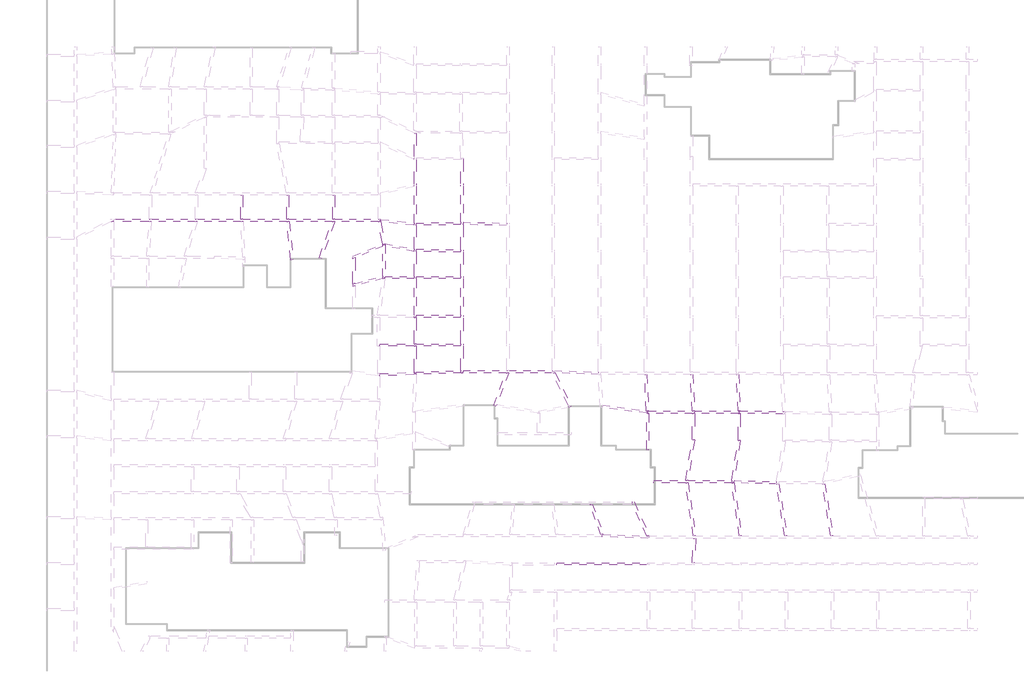
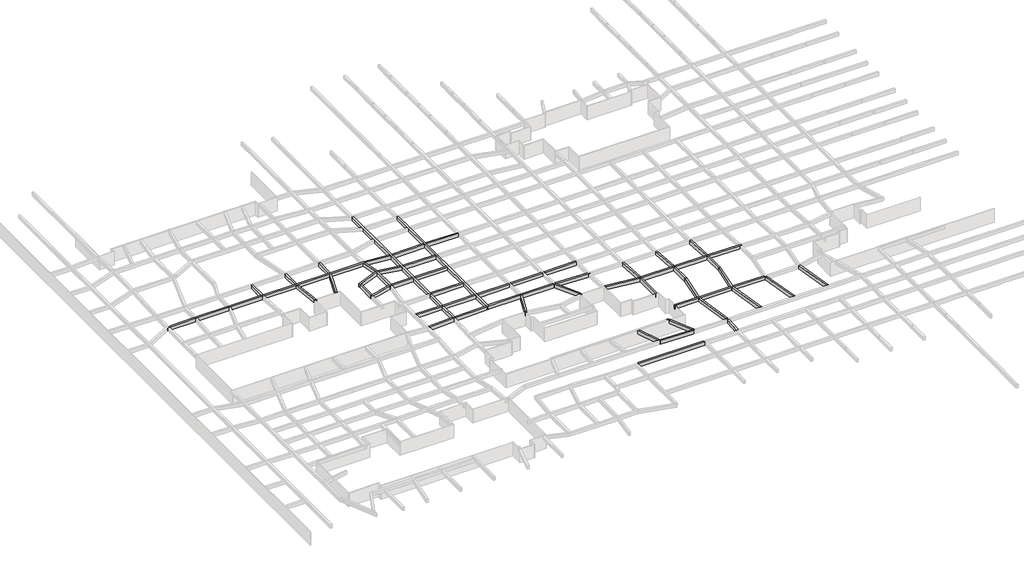
# One storey, part 20 of 45: 53 beams.
"""IFC4 building model written with IfcOpenShell, lengths in millimetres."""

from ifc_helpers import new_model, si_unit, frame, origin, place, context, project, spatial, polyline, outline, extrude, faceted_brep, element, save

model = new_model("IFC4")

# Units and contexts
model_context = context("Model", 3, world=origin())
ifc_project = project(units=[si_unit("LENGTHUNIT", "METRE", prefix="MILLI")], contexts=[model_context])

# Site, building, storey
site = spatial("IfcSite", under=ifc_project)
building = spatial("IfcBuilding", under=site)
storey = spatial("IfcBuildingStorey", under=building, Name="户型图", Elevation=0.0)

# Beams
placement = place(None, origin())
element("IfcBeam", 1, ObjectType="混凝土 - 矩形梁 : KL_beam", at=placement, inside=storey, context=model_context, shape_type="Brep", body=[
    faceted_brep([(-98412.8771817, -3306.533538, 3300.0), (-98412.8771817, -3089.2020745, 3300.0), (-98412.8771817, -2926.5480751, 3300.0), (-98412.8771817, -2906.533538, 3300.0), (-98812.8771817, -2906.533538, 3300.0), (-106143.1610176, -2906.533538, 3300.0), (-106543.1610176, -2906.533538, 3300.0), (-113943.1610176, -2906.533538, 3300.0), (-114343.1610176, -2906.533538, 3300.0), (-121743.1610176, -2906.533538, 3300.0), (-122143.1610176, -2906.533538, 3300.0), (-129467.9283627, -2906.533538, 3300.0), (-129867.9283627, -2906.533538, 3300.0), (-137267.9283627, -2906.533538, 3300.0), (-137667.9283627, -2906.533538, 3300.0), (-143362.5840071, -2906.533538, 3300.0), (-144147.6282093, -3306.533538, 3300.0), (-144104.0852782, -3306.533538, 3300.0), (-143704.0852782, -3306.533538, 3300.0), (-137682.4021047, -3306.533538, 3300.0), (-137281.4253454, -3306.533538, 3300.0), (-129938.2128502, -3306.533538, 3300.0), (-129519.9361477, -3306.533538, 3300.0), (-122132.953931, -3306.533538, 3300.0), (-121732.4049926, -3306.533538, 3300.0), (-114323.2418265, -3306.533538, 3300.0), (-113921.0385147, -3306.533538, 3300.0), (-106625.5164731, -3306.533538, 3300.0), (-106201.4956125, -3306.533538, 3300.0), (-98778.0584965, -3306.533538, 3300.0), (-98412.8771817, -2906.533538, 2500.0), (-98812.8771817, -2906.533538, 2500.0), (-106143.1610176, -2906.533538, 2500.0), (-106543.1610176, -2906.533538, 2500.0), (-113943.1610176, -2906.533538, 2500.0), (-114343.1610176, -2906.533538, 2500.0), (-121743.1610176, -2906.533538, 2500.0), (-122143.1610176, -2906.533538, 2500.0), (-129467.9283627, -2906.533538, 2500.0), (-129867.9283627, -2906.533538, 2500.0), (-137267.9283627, -2906.533538, 2500.0), (-137667.9283627, -2906.533538, 2500.0), (-143362.5840071, -2906.533538, 2500.0), (-98412.8771817, -2926.5480751, 2500.0), (-98412.8771817, -3089.2020745, 2500.0), (-98412.8771817, -3306.533538, 2500.0), (-98778.0584965, -3306.533538, 2500.0), (-106201.4956125, -3306.533538, 2500.0), (-106625.5164731, -3306.533538, 2500.0), (-113921.0385147, -3306.533538, 2500.0), (-114323.2418265, -3306.533538, 2500.0), (-121732.4049926, -3306.533538, 2500.0), (-122132.953931, -3306.533538, 2500.0), (-129519.9361477, -3306.533538, 2500.0), (-129938.2128502, -3306.533538, 2500.0), (-137281.4253454, -3306.533538, 2500.0), (-137682.4021047, -3306.533538, 2500.0), (-143704.0852782, -3306.533538, 2500.0), (-144104.0852782, -3306.533538, 2500.0), (-144147.6282093, -3306.533538, 2500.0)], [[[0, 1, 2, 3, 4, 5, 6, 7, 8, 9, 10, 11, 12, 13, 14, 15, 16, 17, 18, 19, 20, 21, 22, 23, 24, 25, 26, 27, 28, 29]], [[3, 30, 31, 32, 33, 34, 35, 36, 37, 38, 39, 40, 41, 42, 15, 14, 13, 12, 11, 10, 9, 8, 7, 6, 5, 4]], [[30, 43, 44, 45, 46, 47, 48, 49, 50, 51, 52, 53, 54, 55, 56, 57, 58, 59, 42, 41, 40, 39, 38, 37, 36, 35, 34, 33, 32, 31]], [[45, 0, 29, 28, 27, 26, 25, 24, 23, 22, 21, 20, 19, 18, 17, 16, 59, 58, 57, 56, 55, 54, 53, 52, 51, 50, 49, 48, 47, 46]], [[16, 15, 42, 59]], [[3, 2, 1, 0, 45, 44, 43, 30]]]),
])
element("IfcBeam", 2, ObjectType="混凝土 - 矩形梁 : KL_beam", at=placement, inside=storey, context=model_context, shape_type="Brep", body=[
    faceted_brep([(-92291.6701424, 11700.217385, 3300.0), (-92534.6339278, 11700.217385, 3300.0), (-92691.6701424, 11770.1344124, 3300.0), (-92691.6701424, 7708.1903778, 3300.0), (-92691.6701424, 7270.3358664, 3300.0), (-92691.6701424, 3075.9119134, 3300.0), (-92691.6701424, 2663.6664617, 3300.0), (-92691.6701424, -3530.9179057, 3300.0), (-92691.6701424, -3933.1435393, 3300.0), (-92691.6701424, -7966.4140235, 3300.0), (-92691.6701424, -8373.1172498, 3300.0), (-92691.6701424, -12606.533538, 3300.0), (-92691.6701424, -13006.533538, 3300.0), (-92691.6701424, -19206.533538, 3300.0), (-92691.6701424, -19606.533538, 3300.0), (-92291.6701424, -19606.533538, 3300.0), (-92291.6701424, -19566.2432363, 3300.0), (-92291.6701424, -19166.2432363, 3300.0), (-92291.6701424, -13006.533538, 3300.0), (-92291.6701424, -12606.533538, 3300.0), (-92291.6701424, -8372.0681142, 3300.0), (-92291.6701424, -7972.007183, 3300.0), (-92291.6701424, -3949.6812515, 3300.0), (-92291.6701424, -3549.6203203, 3300.0), (-92291.6701424, 2719.5822838, 3300.0), (-92291.6701424, 3119.5822838, 3300.0), (-92291.6701424, 7200.318112, 3300.0), (-92291.6701424, 7600.318112, 3300.0), (-92691.6701424, 11770.1344124, 2500.0), (-92691.6701424, 7708.1903778, 2500.0), (-92691.6701424, 7270.3358664, 2500.0), (-92691.6701424, 3075.9119134, 2500.0), (-92691.6701424, 2663.6664617, 2500.0), (-92691.6701424, -3530.9179057, 2500.0), (-92691.6701424, -3933.1435393, 2500.0), (-92691.6701424, -7966.4140235, 2500.0), (-92691.6701424, -8373.1172498, 2500.0), (-92691.6701424, -12606.533538, 2500.0), (-92691.6701424, -13006.533538, 2500.0), (-92691.6701424, -19206.533538, 2500.0), (-92691.6701424, -19606.533538, 2500.0), (-92534.6339278, 11700.217385, 2500.0), (-92291.6701424, 11700.217385, 2500.0), (-92291.6701424, 7600.318112, 2500.0), (-92291.6701424, 7200.318112, 2500.0), (-92291.6701424, 3119.5822838, 2500.0), (-92291.6701424, 2719.5822838, 2500.0), (-92291.6701424, -3549.6203203, 2500.0), (-92291.6701424, -3949.6812515, 2500.0), (-92291.6701424, -7972.007183, 2500.0), (-92291.6701424, -8372.0681142, 2500.0), (-92291.6701424, -12606.533538, 2500.0), (-92291.6701424, -13006.533538, 2500.0), (-92291.6701424, -19166.2432363, 2500.0), (-92291.6701424, -19566.2432363, 2500.0), (-92291.6701424, -19606.533538, 2500.0)], [[[0, 1, 2, 3, 4, 5, 6, 7, 8, 9, 10, 11, 12, 13, 14, 15, 16, 17, 18, 19, 20, 21, 22, 23, 24, 25, 26, 27]], [[2, 28, 29, 30, 31, 32, 33, 34, 35, 36, 37, 38, 39, 40, 14, 13, 12, 11, 10, 9, 8, 7, 6, 5, 4, 3]], [[41, 42, 43, 44, 45, 46, 47, 48, 49, 50, 51, 52, 53, 54, 55, 40, 39, 38, 37, 36, 35, 34, 33, 32, 31, 30, 29, 28]], [[42, 0, 27, 26, 25, 24, 23, 22, 21, 20, 19, 18, 17, 16, 15, 55, 54, 53, 52, 51, 50, 49, 48, 47, 46, 45, 44, 43]], [[41, 1, 0, 42]], [[1, 41, 28, 2]], [[15, 14, 40, 55]]]),
])
element("IfcBeam", 3, ObjectType="混凝土 - 矩形梁 : KL_beam", at=placement, inside=storey, context=model_context, shape_type="SweptSolid", body=[
    extrude(outline(polyline([(-121743.1610176, -2906.533538), (-122143.1610176, -2906.533538), (-122143.1610176, 1193.466462), (-121743.1610176, 1193.466462), (-121743.1610176, -2906.533538)])), frame((0.0, 0.0, 2500.0), z_axis=(0.0, 0.0, 1.0), x_axis=(1.0, 0.0, 0.0)), (0.0, 0.0, 1.0), 800.0),
])
element("IfcBeam", 4, ObjectType="混凝土 - 矩形梁 : KL_beam", at=placement, inside=storey, context=model_context, shape_type="SweptSolid", body=[
    extrude(outline(polyline([(-113943.1610176, -2906.533538), (-114343.1610176, -2906.533538), (-114343.1610176, 1193.466462), (-113943.1610176, 1193.466462), (-113943.1610176, -2906.533538)])), frame((0.0, 0.0, 2500.0), z_axis=(0.0, 0.0, 1.0), x_axis=(1.0, 0.0, 0.0)), (0.0, 0.0, 1.0), 800.0),
])
element("IfcBeam", 5, ObjectType="混凝土 - 矩形梁 : KL_beam", at=placement, inside=storey, context=model_context, shape_type="SweptSolid", body=[
    extrude(outline(polyline([(-106143.1610176, -2906.533538), (-106543.1610176, -2906.533538), (-106543.1610176, 1193.466462), (-106143.1610176, 1193.466462), (-106143.1610176, -2906.533538)])), frame((0.0, 0.0, 2500.0), z_axis=(0.0, 0.0, 1.0), x_axis=(1.0, 0.0, 0.0)), (0.0, 0.0, 1.0), 800.0),
])
element("IfcBeam", 6, ObjectType="混凝土 - 矩形梁 : KL_beam", at=placement, inside=storey, context=model_context, shape_type="SweptSolid", body=[
    extrude(outline(polyline([(-113240.416887, -9782.2157591), (-113638.2256451, -9824.0271444), (-114323.2418265, -3306.533538), (-113921.0385147, -3306.533538), (-113240.416887, -9782.2157591)])), frame((0.0, 0.0, 2500.0), z_axis=(0.0, 0.0, 1.0), x_axis=(1.0, 0.0, 0.0)), (0.0, 0.0, 1.0), 800.0),
])
element("IfcBeam", 7, ObjectType="混凝土 - 矩形梁 : KL_beam", at=placement, inside=storey, context=model_context, shape_type="SweptSolid", body=[
    extrude(outline(polyline([(-108410.7299112, -9587.6722396), (-108788.0698368, -9454.9523069), (-106625.5164731, -3306.533538), (-106201.4956125, -3306.533538), (-108410.7299112, -9587.6722396)])), frame((0.0, 0.0, 2500.0), z_axis=(0.0, 0.0, 1.0), x_axis=(1.0, 0.0, 0.0)), (0.0, 0.0, 1.0), 800.0),
])
element("IfcBeam", 8, ObjectType="混凝土 - 矩形梁 : KL_beam", at=placement, inside=storey, context=model_context, shape_type="Brep", body=[
    faceted_brep([(-97610.1601463, -7209.73689, 3300.0), (-97639.9689694, -7056.7212093, 3300.0), (-98365.2258689, -3333.8074395, 3300.0), (-98412.8771817, -3089.2020745, 3300.0), (-98412.8771817, -3306.533538, 3300.0), (-98778.0584965, -3306.533538, 3300.0), (-98038.0080665, -7105.3859697, 3300.0), (-98010.1601463, -7248.3358759, 3300.0), (-98778.0584965, -3306.533538, 2500.0), (-98038.0080665, -7105.3859697, 2500.0), (-98010.1601463, -7248.3358759, 2500.0), (-98412.8771817, -3306.533538, 2500.0), (-98412.8771817, -3089.2020745, 2500.0), (-98365.2258689, -3333.8074395, 2500.0), (-97639.9689694, -7056.7212093, 2500.0), (-97610.1601463, -7209.73689, 2500.0)], [[[0, 1, 2, 3, 4, 5, 6, 7]], [[7, 6, 5, 8, 9, 10]], [[10, 9, 8, 11, 12, 13, 14, 15]], [[3, 2, 1, 0, 15, 14, 13, 12]], [[4, 11, 8, 5]], [[11, 4, 3, 12]], [[0, 7, 10, 15]]]),
])
element("IfcBeam", 9, ObjectType="混凝土 - 矩形梁 : KL_beam", at=placement, inside=storey, context=model_context, shape_type="Brep", body=[
    faceted_brep([(-97610.1601463, -7209.73689, 3300.0), (-98010.1601463, -7248.3358759, 3300.0), (-98010.1601463, -7525.5485767, 3300.0), (-98010.1601463, -12553.0681404, 3300.0), (-98010.1601463, -12967.1786125, 3300.0), (-97610.1601463, -12859.9989355, 3300.0), (-97610.1601463, -12606.533538, 3300.0), (-97610.1601463, -7468.9044749, 3300.0), (-97610.1601463, -7363.9380863, 3300.0), (-98010.1601463, -7248.3358759, 2500.0), (-98010.1601463, -7525.5485767, 2500.0), (-98010.1601463, -12553.0681404, 2500.0), (-98010.1601463, -12967.1786125, 2500.0), (-97610.1601463, -7209.73689, 2500.0), (-97610.1601463, -7363.9380863, 2500.0), (-97610.1601463, -7468.9044749, 2500.0), (-97610.1601463, -12606.533538, 2500.0), (-97610.1601463, -12859.9989355, 2500.0)], [[[0, 1, 2, 3, 4, 5, 6, 7, 8]], [[1, 9, 10, 11, 12, 4, 3, 2]], [[9, 13, 14, 15, 16, 17, 12, 11, 10]], [[13, 0, 8, 7, 6, 5, 17, 16, 15, 14]], [[0, 13, 9, 1]], [[5, 4, 12, 17]]]),
])
element("IfcBeam", 10, ObjectType="混凝土 - 矩形梁 : KL_beam", at=placement, inside=storey, context=model_context, shape_type="Brep", body=[
    faceted_brep([(-98010.1601463, -7248.3358759, 3300.0), (-98038.0080665, -7105.3859697, 3300.0), (-103109.6713464, -9154.4709434, 3300.0), (-103109.6713464, -9585.8848405, 3300.0), (-102709.6713464, -9424.2743501, 3300.0), (-98010.1601463, -7525.5485767, 3300.0), (-98038.0080665, -7105.3859697, 2500.0), (-103109.6713464, -9154.4709434, 2500.0), (-98010.1601463, -7248.3358759, 2500.0), (-98010.1601463, -7525.5485767, 2500.0), (-102709.6713464, -9424.2743501, 2500.0), (-103109.6713464, -9585.8848405, 2500.0)], [[[0, 1, 2, 3, 4, 5]], [[1, 6, 7, 2]], [[6, 8, 9, 10, 11, 7]], [[3, 11, 10, 9, 5, 4]], [[1, 0, 8, 6]], [[0, 5, 9, 8]], [[3, 2, 7, 11]]]),
    faceted_brep([(-97582.312226, -7352.6867962, 3300.0), (-97582.312226, -7352.6867962, 2500.0), (-97610.1601463, -7209.73689, 2500.0), (-97610.1601463, -7209.73689, 3300.0), (-97610.1601463, -7363.9380863, 3300.0), (-97610.1601463, -7363.9380863, 2500.0)], [[[0, 1, 2, 3]], [[4, 3, 2, 5]], [[0, 3, 4]], [[2, 1, 5]], [[1, 0, 4, 5]]]),
])
element("IfcBeam", 11, ObjectType="混凝土 - 矩形梁 : KL_beam", at=placement, inside=storey, context=model_context, shape_type="Brep", body=[
    faceted_brep([(-103109.6713464, -13919.4780482, 3300.0), (-103006.1437284, -14305.8483787, 3300.0), (-102709.6713464, -14226.4088434, 3300.0), (-98050.230566, -12977.9154491, 3300.0), (-98010.1601463, -12967.1786125, 3300.0), (-98010.1601463, -12553.0681404, 3300.0), (-102709.6713464, -13812.2983712, 3300.0), (-103109.6713464, -13919.4780482, 2500.0), (-98010.1601463, -12553.0681404, 2500.0), (-102709.6713464, -13812.2983712, 2500.0), (-103006.1437284, -14305.8483787, 2500.0), (-98010.1601463, -12967.1786125, 2500.0), (-98050.230566, -12977.9154491, 2500.0), (-102709.6713464, -14226.4088434, 2500.0)], [[[0, 1, 2, 3, 4, 5, 6]], [[7, 0, 6, 5, 8, 9]], [[10, 7, 9, 8, 11, 12, 13]], [[1, 10, 13, 12, 11, 4, 3, 2]], [[5, 4, 11, 8]], [[1, 0, 7, 10]]]),
])
element("IfcBeam", 12, ObjectType="混凝土 - 矩形梁 : KL_beam", at=placement, inside=storey, context=model_context, shape_type="SweptSolid", body=[
    extrude(outline(polyline([(-103109.6713464, -13919.4780482), (-103109.6713464, -9585.8848405), (-102709.6713464, -9424.2743501), (-102709.6713464, -13812.2983712), (-103109.6713464, -13919.4780482)])), frame((0.0, 0.0, 2500.0), z_axis=(0.0, 0.0, 1.0), x_axis=(1.0, 0.0, 0.0)), (0.0, 0.0, 1.0), 800.0),
])
element("IfcBeam", 13, ObjectType="混凝土 - 矩形梁 : KL_beam", at=placement, inside=storey, context=model_context, shape_type="Brep", body=[
    faceted_brep([(-98010.1601463, -13006.533538, 3300.0), (-97650.3215471, -13006.533538, 3300.0), (-92691.6701424, -13006.533538, 3300.0), (-92691.6701424, -12606.533538, 3300.0), (-97610.1601463, -12606.533538, 3300.0), (-97610.1601463, -12859.9989355, 3300.0), (-98010.1601463, -12967.1786125, 3300.0), (-92691.6701424, -12606.533538, 2500.0), (-97610.1601463, -12606.533538, 2500.0), (-92691.6701424, -13006.533538, 2500.0), (-97650.3215471, -13006.533538, 2500.0), (-98010.1601463, -13006.533538, 2500.0), (-98010.1601463, -12967.1786125, 2500.0), (-97610.1601463, -12859.9989355, 2500.0)], [[[0, 1, 2, 3, 4, 5, 6]], [[3, 7, 8, 4]], [[9, 10, 11, 12, 13, 8, 7]], [[0, 11, 10, 9, 2, 1]], [[11, 0, 6, 12]], [[3, 2, 9, 7]], [[5, 13, 12, 6]], [[13, 5, 4, 8]]]),
])
element("IfcBeam", 14, ObjectType="混凝土 - 矩形梁 : KL_beam", at=placement, inside=storey, context=model_context, shape_type="Brep", body=[
    faceted_brep([(-92691.6701424, -8373.1172498, 3300.0), (-92691.6701424, -7966.4140235, 3300.0), (-97639.9689694, -7056.7212093, 3300.0), (-97610.1601463, -7209.73689, 3300.0), (-97582.312226, -7352.6867962, 3300.0), (-97610.1601463, -7363.9380863, 3300.0), (-97610.1601463, -7468.9044749, 3300.0), (-92691.6701424, -7966.4140235, 2500.0), (-97639.9689694, -7056.7212093, 2500.0), (-92691.6701424, -8373.1172498, 2500.0), (-97610.1601463, -7468.9044749, 2500.0), (-97610.1601463, -7363.9380863, 2500.0), (-97582.312226, -7352.6867962, 2500.0), (-97610.1601463, -7209.73689, 2500.0)], [[[0, 1, 2, 3, 4, 5, 6]], [[1, 7, 8, 2]], [[7, 9, 10, 11, 12, 13, 8]], [[9, 0, 6, 10]], [[1, 0, 9, 7]], [[2, 8, 13, 12, 4, 3]], [[10, 6, 5, 11]], [[4, 12, 11, 5]]]),
])
element("IfcBeam", 15, ObjectType="混凝土 - 矩形梁 : KL_beam", at=placement, inside=storey, context=model_context, shape_type="SweptSolid", body=[
    extrude(outline(polyline([(-98412.8771817, -2926.5480751), (-92691.6701424, -3530.9179057), (-92691.6701424, -3933.1435393), (-98365.2258689, -3333.8074395), (-98412.8771817, -3089.2020745), (-98412.8771817, -2926.5480751)])), frame((0.0, 0.0, 2500.0), z_axis=(0.0, 0.0, 1.0), x_axis=(1.0, 0.0, 0.0)), (0.0, 0.0, 1.0), 800.0),
])
element("IfcBeam", 16, ObjectType="混凝土 - 矩形梁 : KL_beam", at=placement, inside=storey, context=model_context, shape_type="Brep", body=[
    faceted_brep([(-84386.4058027, 7406.4496764, 3300.0), (-84786.4058027, 7399.4676504, 3300.0), (-84786.4058027, 7200.318112, 3300.0), (-84786.4058027, 3119.5822838, 3300.0), (-84786.4058027, 2719.5822838, 3300.0), (-84786.4058027, -3418.615444, 3300.0), (-84786.4058027, -3818.6763752, 3300.0), (-84786.4058027, -8103.0120594, 3300.0), (-84786.4058027, -8503.0729906, 3300.0), (-84786.4058027, -12606.533538, 3300.0), (-84786.4058027, -13006.533538, 3300.0), (-84786.4058027, -19166.2432363, 3300.0), (-84786.4058027, -19566.2432363, 3300.0), (-84786.4058027, -24066.2432363, 3300.0), (-84786.4058027, -24466.2432363, 3300.0), (-84786.4058027, -28603.7362156, 3300.0), (-84786.4058027, -29003.9680843, 3300.0), (-84583.0013827, -28997.0413366, 3300.0), (-84386.4058027, -28990.3464576, 3300.0), (-84386.4058027, -28597.0413366, 3300.0), (-84386.4058027, -24466.2432363, 3300.0), (-84386.4058027, -24066.2432363, 3300.0), (-84386.4058027, -19666.2432363, 3300.0), (-84386.4058027, -19266.2432363, 3300.0), (-84386.4058027, -13006.533538, 3300.0), (-84386.4058027, -12606.533538, 3300.0), (-84386.4058027, -8506.533538, 3300.0), (-84386.4058027, -8106.533538, 3300.0), (-84386.4058027, -3818.6763752, 3300.0), (-84386.4058027, -3418.615444, 3300.0), (-84386.4058027, 2719.5822838, 3300.0), (-84386.4058027, 3119.5822838, 3300.0), (-84386.4058027, 7200.318112, 3300.0), (-84786.4058027, 7399.4676504, 2500.0), (-84786.4058027, 7200.318112, 2500.0), (-84786.4058027, 3119.5822838, 2500.0), (-84786.4058027, 2719.5822838, 2500.0), (-84786.4058027, -3418.615444, 2500.0), (-84786.4058027, -3818.6763752, 2500.0), (-84786.4058027, -8103.0120594, 2500.0), (-84786.4058027, -8503.0729906, 2500.0), (-84786.4058027, -12606.533538, 2500.0), (-84786.4058027, -13006.533538, 2500.0), (-84786.4058027, -19166.2432363, 2500.0), (-84786.4058027, -19566.2432363, 2500.0), (-84786.4058027, -24066.2432363, 2500.0), (-84786.4058027, -24466.2432363, 2500.0), (-84786.4058027, -28603.7362156, 2500.0), (-84786.4058027, -29003.9680843, 2500.0), (-84386.4058027, 7406.4496764, 2500.0), (-84386.4058027, 7200.318112, 2500.0), (-84386.4058027, 3119.5822838, 2500.0), (-84386.4058027, 2719.5822838, 2500.0), (-84386.4058027, -3418.615444, 2500.0), (-84386.4058027, -3818.6763752, 2500.0), (-84386.4058027, -8106.533538, 2500.0), (-84386.4058027, -8506.533538, 2500.0), (-84386.4058027, -12606.533538, 2500.0), (-84386.4058027, -13006.533538, 2500.0), (-84386.4058027, -19266.2432363, 2500.0), (-84386.4058027, -19666.2432363, 2500.0), (-84386.4058027, -24066.2432363, 2500.0), (-84386.4058027, -24466.2432363, 2500.0), (-84386.4058027, -28597.0413366, 2500.0), (-84386.4058027, -28990.3464576, 2500.0), (-84583.0013827, -28997.0413366, 2500.0)], [[[0, 1, 2, 3, 4, 5, 6, 7, 8, 9, 10, 11, 12, 13, 14, 15, 16, 17, 18, 19, 20, 21, 22, 23, 24, 25, 26, 27, 28, 29, 30, 31, 32]], [[1, 33, 34, 35, 36, 37, 38, 39, 40, 41, 42, 43, 44, 45, 46, 47, 48, 16, 15, 14, 13, 12, 11, 10, 9, 8, 7, 6, 5, 4, 3, 2]], [[33, 49, 50, 51, 52, 53, 54, 55, 56, 57, 58, 59, 60, 61, 62, 63, 64, 65, 48, 47, 46, 45, 44, 43, 42, 41, 40, 39, 38, 37, 36, 35, 34]], [[49, 0, 32, 31, 30, 29, 28, 27, 26, 25, 24, 23, 22, 21, 20, 19, 18, 64, 63, 62, 61, 60, 59, 58, 57, 56, 55, 54, 53, 52, 51, 50]], [[0, 49, 33, 1]], [[18, 17, 16, 48, 65, 64]]]),
])
element("IfcBeam", 17, ObjectType="混凝土 - 矩形梁 : KL_beam", at=placement, inside=storey, context=model_context, shape_type="SweptSolid", body=[
    extrude(outline(polyline([(-92291.6701424, -3949.6812515), (-92291.6701424, -3549.6203203), (-84786.4058027, -3418.615444), (-84786.4058027, -3818.6763752), (-92291.6701424, -3949.6812515)])), frame((0.0, 0.0, 2500.0), z_axis=(0.0, 0.0, 1.0), x_axis=(1.0, 0.0, 0.0)), (0.0, 0.0, 1.0), 800.0),
])
element("IfcBeam", 18, ObjectType="混凝土 - 矩形梁 : KL_beam", at=placement, inside=storey, context=model_context, shape_type="SweptSolid", body=[
    extrude(outline(polyline([(-76974.0592951, -3547.9984335), (-76974.0592951, -3948.0593648), (-84386.4058027, -3818.6763752), (-84386.4058027, -3418.615444), (-76974.0592951, -3547.9984335)])), frame((0.0, 0.0, 2500.0), z_axis=(0.0, 0.0, 1.0), x_axis=(1.0, 0.0, 0.0)), (0.0, 0.0, 1.0), 800.0),
])
element("IfcBeam", 19, ObjectType="混凝土 - 矩形梁 : KL_beam", at=placement, inside=storey, context=model_context, shape_type="SweptSolid", body=[
    extrude(outline(polyline([(-92291.6701424, -8372.0681142), (-92291.6701424, -7972.007183), (-84786.4058027, -8103.0120594), (-84786.4058027, -8503.0729906), (-92291.6701424, -8372.0681142)])), frame((0.0, 0.0, 2500.0), z_axis=(0.0, 0.0, 1.0), x_axis=(1.0, 0.0, 0.0)), (0.0, 0.0, 1.0), 800.0),
])
element("IfcBeam", 20, ObjectType="混凝土 - 矩形梁 : KL_beam", at=placement, inside=storey, context=model_context, shape_type="SweptSolid", body=[
    extrude(outline(polyline([(-92291.6701424, -13006.533538), (-92291.6701424, -12606.533538), (-84786.4058027, -12606.533538), (-84786.4058027, -13006.533538), (-92291.6701424, -13006.533538)])), frame((0.0, 0.0, 2500.0), z_axis=(0.0, 0.0, 1.0), x_axis=(1.0, 0.0, 0.0)), (0.0, 0.0, 1.0), 800.0),
])
element("IfcBeam", 21, ObjectType="混凝土 - 矩形梁 : KL_beam", at=placement, inside=storey, context=model_context, shape_type="SweptSolid", body=[
    extrude(outline(polyline([(-92291.6701424, -19566.2432363), (-92291.6701424, -19166.2432363), (-84786.4058027, -19166.2432363), (-84786.4058027, -19566.2432363), (-92291.6701424, -19566.2432363)])), frame((0.0, 0.0, 2500.0), z_axis=(0.0, 0.0, 1.0), x_axis=(1.0, 0.0, 0.0)), (0.0, 0.0, 1.0), 800.0),
])
element("IfcBeam", 22, ObjectType="混凝土 - 矩形梁 : KL_beam", at=placement, inside=storey, context=model_context, shape_type="SweptSolid", body=[
    extrude(outline(polyline([(-92691.5379725, -19606.533538), (-92291.5379725, -19606.533538), (-92291.5379725, -24066.2432363), (-92691.5379725, -24066.2432363), (-92691.5379725, -19606.533538)])), frame((0.0, 0.0, 2500.0), z_axis=(0.0, 0.0, 1.0), x_axis=(1.0, 0.0, 0.0)), (0.0, 0.0, 1.0), 800.0),
])
element("IfcBeam", 23, ObjectType="混凝土 - 矩形梁 : KL_beam", at=placement, inside=storey, context=model_context, shape_type="Brep", body=[
    faceted_brep([(-98551.6884215, -24066.2432363, 3300.0), (-98551.6884215, -24466.2432363, 3300.0), (-98489.6882512, -24466.2432363, 3300.0), (-92691.5379725, -24466.2432363, 3300.0), (-92291.5379725, -24466.2432363, 3300.0), (-84786.4058027, -24466.2432363, 3300.0), (-84786.4058027, -24066.2432363, 3300.0), (-92291.5379725, -24066.2432363, 3300.0), (-92691.5379725, -24066.2432363, 3300.0), (-98551.6884215, -24066.2432363, 2500.0), (-84786.4058027, -24066.2432363, 2500.0), (-92291.5379725, -24066.2432363, 2500.0), (-92691.5379725, -24066.2432363, 2500.0), (-98551.6884215, -24466.2432363, 2500.0), (-84786.4058027, -24466.2432363, 2500.0), (-92291.5379725, -24466.2432363, 2500.0), (-92691.5379725, -24466.2432363, 2500.0), (-98489.6882512, -24466.2432363, 2500.0)], [[[0, 1, 2, 3, 4, 5, 6, 7, 8]], [[9, 0, 8, 7, 6, 10, 11, 12]], [[13, 9, 12, 11, 10, 14, 15, 16, 17]], [[1, 13, 17, 16, 15, 14, 5, 4, 3, 2]], [[1, 0, 9, 13]], [[6, 5, 14, 10]]]),
    faceted_brep([(-61385.2176693, -24066.2432363, 3300.0), (-61385.2176693, -24466.2432363, 3300.0), (-61385.2176693, -24466.2432363, 2500.0), (-61385.2176693, -24066.2432363, 2500.0), (-68859.410716, -24466.2432363, 3300.0), (-68859.410716, -24066.2432363, 3300.0), (-68859.410716, -24066.2432363, 2500.0), (-68859.410716, -24466.2432363, 2500.0)], [[[0, 1, 2, 3]], [[4, 5, 6, 7]], [[1, 0, 5, 4]], [[0, 3, 6, 5]], [[3, 2, 7, 6]], [[2, 1, 4, 7]]]),
    faceted_brep([(-76974.0592951, -24066.2432363, 3300.0), (-76974.0592951, -24466.2432363, 3300.0), (-76974.0592951, -24466.2432363, 2500.0), (-76974.0592951, -24066.2432363, 2500.0), (-84386.4058027, -24466.2432363, 3300.0), (-84386.4058027, -24066.2432363, 3300.0), (-84386.4058027, -24066.2432363, 2500.0), (-84386.4058027, -24466.2432363, 2500.0)], [[[0, 1, 2, 3]], [[4, 5, 6, 7]], [[1, 0, 5, 4]], [[0, 3, 6, 5]], [[3, 2, 7, 6]], [[2, 1, 4, 7]]]),
    faceted_brep([(-76574.0592951, -24466.2432363, 3300.0), (-76574.0592951, -24066.2432363, 3300.0), (-76574.0592951, -24066.2432363, 2500.0), (-76574.0592951, -24466.2432363, 2500.0), (-69259.410716, -24466.2432363, 3300.0), (-69259.410716, -24066.2432363, 3300.0), (-69259.410716, -24066.2432363, 2500.0), (-69259.410716, -24466.2432363, 2500.0)], [[[0, 1, 2, 3]], [[1, 0, 4, 5]], [[2, 1, 5, 6]], [[3, 2, 6, 7]], [[0, 3, 7, 4]], [[5, 4, 7, 6]]]),
])
element("IfcBeam", 24, ObjectType="混凝土 - 矩形梁 : KL_beam", at=placement, inside=storey, context=model_context, shape_type="Brep", body=[
    faceted_brep([(-92691.5379725, -29062.7522233, 3300.0), (-92291.5379725, -29069.7342493, 3300.0), (-92291.5379725, -28859.3164886, 3300.0), (-92291.5379725, -24466.2432363, 3300.0), (-92691.5379725, -24466.2432363, 3300.0), (-92691.5379725, -28874.9728967, 3300.0), (-92691.5379725, -29062.7522233, 2500.0), (-92691.5379725, -24466.2432363, 2500.0), (-92691.5379725, -28874.9728967, 2500.0), (-92291.5379725, -29069.7342493, 2500.0), (-92291.5379725, -24466.2432363, 2500.0), (-92291.5379725, -28859.3164886, 2500.0)], [[[0, 1, 2, 3, 4, 5]], [[6, 0, 5, 4, 7, 8]], [[9, 6, 8, 7, 10, 11]], [[1, 9, 11, 10, 3, 2]], [[4, 3, 10, 7]], [[1, 0, 6, 9]]]),
])
element("IfcBeam", 25, ObjectType="混凝土 - 矩形梁 : KL_beam", at=placement, inside=storey, context=model_context, shape_type="SweptSolid", body=[
    extrude(outline(polyline([(-92691.5379725, -28874.9728967), (-92691.5379725, -29062.7522233), (-92698.9743886, -29275.7033162), (-98489.6882512, -29534.2260627), (-98489.6882512, -29133.8276372), (-92691.5379725, -28874.9728967)])), frame((0.0, 0.0, 2500.0), z_axis=(0.0, 0.0, 1.0), x_axis=(1.0, 0.0, 0.0)), (0.0, 0.0, 1.0), 800.0),
])
element("IfcBeam", 26, ObjectType="混凝土 - 矩形梁 : KL_beam", at=placement, inside=storey, context=model_context, shape_type="Brep", body=[
    faceted_brep([(-84786.4058027, -29003.9680843, 3300.0), (-84786.4058027, -28603.7362156, 3300.0), (-92291.5379725, -28859.3164886, 3300.0), (-92291.5379725, -29069.7342493, 3300.0), (-92298.1056102, -29257.806784, 3300.0), (-92298.1743191, -29259.7743519, 3300.0), (-84786.4058027, -29003.9680843, 2500.0), (-92298.1743191, -29259.7743519, 2500.0), (-84786.4058027, -28603.7362156, 2500.0), (-92298.1056102, -29257.806784, 2500.0), (-92291.5379725, -29069.7342493, 2500.0), (-92291.5379725, -28859.3164886, 2500.0)], [[[0, 1, 2, 3, 4, 5]], [[6, 0, 5, 7]], [[8, 6, 7, 9, 10, 11]], [[1, 8, 11, 2]], [[1, 0, 6, 8]], [[3, 2, 11, 10]], [[7, 5, 4, 3, 10, 9]]]),
])
element("IfcBeam", 27, ObjectType="混凝土 - 矩形梁 : KL_beam", at=placement, inside=storey, context=model_context, shape_type="Brep", body=[
    faceted_brep([(-69259.410716, -28997.0413366, 3300.0), (-69259.410716, -28597.0413366, 3300.0), (-76574.0592951, -28597.0413366, 3300.0), (-76974.0592951, -28597.0413366, 3300.0), (-84386.4058027, -28597.0413366, 3300.0), (-84386.4058027, -28990.3464576, 3300.0), (-84583.0013827, -28997.0413366, 3300.0), (-77065.0611009, -28997.0413366, 3300.0), (-76636.6031034, -28997.0413366, 3300.0), (-69259.410716, -28997.0413366, 2500.0), (-84583.0013827, -28997.0413366, 2500.0), (-77065.0611009, -28997.0413366, 2500.0), (-76636.6031034, -28997.0413366, 2500.0), (-69259.410716, -28597.0413366, 2500.0), (-84386.4058027, -28990.3464576, 2500.0), (-84386.4058027, -28597.0413366, 2500.0), (-76974.0592951, -28597.0413366, 2500.0), (-76574.0592951, -28597.0413366, 2500.0)], [[[0, 1, 2, 3, 4, 5, 6, 7, 8]], [[9, 0, 8, 7, 6, 10, 11, 12]], [[13, 9, 12, 11, 10, 14, 15, 16, 17]], [[1, 13, 17, 16, 15, 4, 3, 2]], [[1, 0, 9, 13]], [[14, 5, 4, 15]], [[5, 14, 10, 6]]]),
])
element("IfcBeam", 28, ObjectType="混凝土 - 矩形梁 : KL_beam", at=placement, inside=storey, context=model_context, shape_type="Brep", body=[
    faceted_brep([(-60985.2176693, -29273.1976575, 3300.0), (-60985.2176693, -29266.2296815, 3300.0), (-60985.2176693, -29259.522509, 3300.0), (-61385.2176693, -29259.522509, 3300.0), (-61375.3451123, -29259.8600307, 3300.0), (-61189.0319378, -29266.2296815, 3300.0), (-60985.2176693, -29273.1976575, 2500.0), (-68733.4619053, -29008.3016795, 3300.0), (-69062.8285047, -28997.0413366, 3300.0), (-69062.8285047, -28997.0413366, 2500.0), (-68733.4619053, -29008.3016795, 2500.0), (-61385.2176693, -29259.522509, 2500.0), (-61375.3451123, -29259.8600307, 2500.0), (-61189.0319378, -29266.2296815, 2500.0), (-60985.2176693, -29259.522509, 2500.0), (-60985.2176693, -29266.2296815, 2500.0), (-68859.410716, -28603.762064, 2500.0), (-68859.410716, -28603.762064, 3300.0), (-61385.2176693, -28859.2888151, 3300.0), (-61385.2176693, -28859.2888151, 2500.0), (-68859.410716, -28997.0413366, 2500.0), (-68859.410716, -28997.0413366, 3300.0)], [[[0, 1, 2, 3, 4, 5]], [[6, 0, 5, 4, 3, 7, 8, 9, 10, 11, 12, 13]], [[14, 15, 6, 13, 12, 11]], [[16, 17, 18, 19]], [[0, 6, 15, 14, 2, 1]], [[20, 21, 17, 16]], [[21, 20, 9, 8]], [[3, 11, 19, 18]], [[11, 3, 2, 14]], [[17, 21, 8, 7, 3, 18]], [[20, 16, 19, 11, 10, 9]]]),
])
element("IfcBeam", 29, ObjectType="混凝土 - 矩形梁 : KL_beam", at=placement, inside=storey, context=model_context, shape_type="Brep", body=[
    faceted_brep([(-45074.9115482, -35866.2296815, 3300.0), (-45074.9115482, -35466.2296815, 3300.0), (-45475.4604866, -35466.2296815, 3300.0), (-52835.3253588, -35466.2296815, 3300.0), (-53012.1394728, -35466.2296815, 3300.0), (-53037.651896, -35866.2296815, 3300.0), (-52825.1182721, -35866.2296815, 3300.0), (-45464.7044616, -35866.2296815, 3300.0), (-45074.9115482, -35866.2296815, 2500.0), (-53037.651896, -35866.2296815, 2500.0), (-52825.1182721, -35866.2296815, 2500.0), (-45464.7044616, -35866.2296815, 2500.0), (-45074.9115482, -35466.2296815, 2500.0), (-53012.1394728, -35466.2296815, 2500.0), (-52835.3253588, -35466.2296815, 2500.0), (-45475.4604866, -35466.2296815, 2500.0)], [[[0, 1, 2, 3, 4, 5, 6, 7]], [[8, 0, 7, 6, 5, 9, 10, 11]], [[12, 8, 11, 10, 9, 13, 14, 15]], [[1, 12, 15, 14, 13, 4, 3, 2]], [[1, 0, 8, 12]], [[4, 13, 9, 5]]]),
])
element("IfcBeam", 30, ObjectType="混凝土 - 矩形梁 : KL_beam", at=placement, inside=storey, context=model_context, shape_type="Brep", body=[
    faceted_brep([(-37472.2975115, -35866.2296815, 3300.0), (-37469.7442944, -35466.2296815, 3300.0), (-37678.745911, -35466.2296815, 3300.0), (-45074.9115482, -35466.2296815, 3300.0), (-45053.9484365, -35866.2296815, 3300.0), (-37667.9878566, -35866.2296815, 3300.0), (-37472.2975115, -35866.2296815, 2500.0), (-45053.9484365, -35866.2296815, 2500.0), (-37667.9878566, -35866.2296815, 2500.0), (-37469.7442944, -35466.2296815, 2500.0), (-45074.9115482, -35466.2296815, 2500.0), (-37678.745911, -35466.2296815, 2500.0)], [[[0, 1, 2, 3, 4, 5]], [[6, 0, 5, 4, 7, 8]], [[9, 6, 8, 7, 10, 11]], [[1, 9, 11, 10, 3, 2]], [[1, 0, 6, 9]], [[4, 3, 10, 7]]]),
])
element("IfcBeam", 31, ObjectType="混凝土 - 矩形梁 : KL_beam", at=placement, inside=storey, context=model_context, shape_type="Brep", body=[
    faceted_brep([(-29669.6887336, -35565.8099149, 3300.0), (-30070.5058465, -35560.6928409, 3300.0), (-37278.0687283, -35468.6767279, 3300.0), (-37469.7442944, -35466.2296815, 3300.0), (-37472.2975115, -35866.2296815, 3300.0), (-37267.9878566, -35868.8380223, 3300.0), (-30059.6078619, -35960.8645671, 3300.0), (-29674.7949597, -35965.7773217, 3300.0), (-37472.2975115, -35866.2296815, 2500.0), (-37267.9878566, -35868.8380223, 2500.0), (-30059.6078619, -35960.8645671, 2500.0), (-29674.7949597, -35965.7773217, 2500.0), (-37469.7442944, -35466.2296815, 2500.0), (-37278.0687283, -35468.6767279, 2500.0), (-30070.5058465, -35560.6928409, 2500.0), (-29669.6887336, -35565.8099149, 2500.0)], [[[0, 1, 2, 3, 4, 5, 6, 7]], [[7, 6, 5, 4, 8, 9, 10, 11]], [[11, 10, 9, 8, 12, 13, 14, 15]], [[3, 2, 1, 0, 15, 14, 13, 12]], [[3, 12, 8, 4]], [[0, 7, 11, 15]]]),
])
element("IfcBeam", 32, ObjectType="混凝土 - 矩形梁 : KL_beam", at=placement, inside=storey, context=model_context, shape_type="SweptSolid", body=[
    extrude(outline(polyline([(-37278.0687283, -35468.6767279), (-37469.7442944, -35466.2296815), (-37678.745911, -35466.2296815), (-38003.6741425, -29266.2296815), (-37783.4522617, -29266.2296815), (-37603.004472, -29268.5333873), (-37278.0687283, -35468.6767279)])), frame((0.0, 0.0, 2500.0), z_axis=(0.0, 0.0, 1.0), x_axis=(1.0, 0.0, 0.0)), (0.0, 0.0, 1.0), 800.0),
])
element("IfcBeam", 33, ObjectType="混凝土 - 矩形梁 : KL_beam", at=placement, inside=storey, context=model_context, shape_type="Brep", body=[
    faceted_brep([(-37267.9878566, -40482.0087446, 3300.0), (-37267.9878566, -35868.8380223, 3300.0), (-37472.2975115, -35866.2296815, 3300.0), (-37657.7827992, -35866.2296815, 3300.0), (-37667.9878566, -35866.2296815, 3300.0), (-37667.9878566, -40450.5280619, 3300.0), (-37667.9878566, -35866.2296815, 2500.0), (-37667.9878566, -40450.5280619, 2500.0), (-37267.9878566, -35868.8380223, 2500.0), (-37267.9878566, -40482.0087446, 2500.0), (-37657.7827992, -35866.2296815, 2500.0), (-37472.2975115, -35866.2296815, 2500.0)], [[[0, 1, 2, 3, 4, 5]], [[5, 4, 6, 7]], [[8, 9, 7, 6, 10, 11]], [[1, 0, 9, 8]], [[2, 1, 8, 11]], [[6, 4, 3, 2, 11, 10]], [[0, 5, 7, 9]]]),
])
element("IfcBeam", 34, ObjectType="混凝土 - 矩形梁 : KL_beam", at=placement, inside=storey, context=model_context, shape_type="Brep", body=[
    faceted_brep([(-37267.9878566, -40482.0087446, 3300.0), (-37667.9878566, -40450.5280619, 3300.0), (-38754.197381, -47308.5850923, 3300.0), (-38817.5511572, -47708.5850923, 3300.0), (-38757.2703802, -47708.5850923, 3300.0), (-38585.5681986, -47708.5850923, 3300.0), (-38412.5651069, -47708.5850923, 3300.0), (-38350.0121941, -47313.6415444, 3300.0), (-37667.9878566, -40450.5280619, 2500.0), (-38754.197381, -47308.5850923, 2500.0), (-38817.5511572, -47708.5850923, 2500.0), (-37267.9878566, -40482.0087446, 2500.0), (-38350.0121941, -47313.6415444, 2500.0), (-38412.5651069, -47708.5850923, 2500.0), (-38585.5681986, -47708.5850923, 2500.0), (-38757.2703802, -47708.5850923, 2500.0)], [[[0, 1, 2, 3, 4, 5, 6, 7]], [[1, 8, 9, 10, 3, 2]], [[8, 11, 12, 13, 14, 15, 10, 9]], [[11, 0, 7, 6, 13, 12]], [[0, 11, 8, 1]], [[6, 5, 4, 3, 10, 15, 14, 13]]]),
])
element("IfcBeam", 35, ObjectType="混凝土 - 矩形梁 : KL_beam", at=placement, inside=storey, context=model_context, shape_type="Brep", body=[
    faceted_brep([(-45475.4604866, -35466.2296815, 3300.0), (-45074.9115482, -35466.2296815, 3300.0), (-45399.8397798, -29266.2296815, 3300.0), (-45800.3887182, -29266.2296815, 3300.0), (-45475.4604866, -35466.2296815, 2500.0), (-45800.3887182, -29266.2296815, 2500.0), (-45074.9115482, -35466.2296815, 2500.0), (-45399.8397798, -29266.2296815, 2500.0), (-45053.9484365, -35866.2296815, 3300.0), (-45053.9484365, -35866.2296815, 2500.0), (-45064.7044616, -35866.2296815, 3300.0), (-45074.9115482, -35866.2296815, 3300.0), (-45074.9115482, -35866.2296815, 2500.0), (-45064.7044616, -35866.2296815, 2500.0)], [[[0, 1, 2, 3]], [[4, 0, 3, 5]], [[6, 4, 5, 7]], [[8, 9, 6, 7, 2, 1]], [[9, 8, 10, 11, 12, 13]], [[6, 1, 0, 4]], [[1, 6, 12, 11]], [[11, 10, 8, 1]], [[9, 13, 12, 6]], [[3, 2, 7, 5]]]),
])
element("IfcBeam", 36, ObjectType="混凝土 - 矩形梁 : KL_beam", at=placement, inside=storey, context=model_context, shape_type="Brep", body=[
    faceted_brep([(-45464.7044616, -35866.2296815, 3300.0), (-45464.7044616, -40350.4893402, 3300.0), (-45064.7044616, -40381.9700229, 3300.0), (-45064.7044616, -35866.2296815, 3300.0), (-45074.9115482, -35866.2296815, 3300.0), (-45464.7044616, -35866.2296815, 2500.0), (-45464.7044616, -40350.4893402, 2500.0), (-45074.9115482, -35866.2296815, 2500.0), (-45064.7044616, -35866.2296815, 2500.0), (-45064.7044616, -40381.9700229, 2500.0)], [[[0, 1, 2, 3, 4]], [[1, 0, 5, 6]], [[6, 5, 7, 8, 9]], [[3, 2, 9, 8]], [[5, 0, 4, 3, 8, 7]], [[2, 1, 6, 9]]]),
])
element("IfcBeam", 37, ObjectType="混凝土 - 矩形梁 : KL_beam", at=placement, inside=storey, context=model_context, shape_type="SweptSolid", body=[
    extrude(outline(polyline([(-45464.7044616, -40350.4893402), (-45064.7044616, -40381.9700229), (-46161.7725127, -47308.5850923), (-46566.758563, -47308.5850923), (-45464.7044616, -40350.4893402)])), frame((0.0, 0.0, 2500.0), z_axis=(0.0, 0.0, 1.0), x_axis=(1.0, 0.0, 0.0)), (0.0, 0.0, 1.0), 800.0),
])
element("IfcBeam", 38, ObjectType="混凝土 - 矩形梁 : KL_beam", at=placement, inside=storey, context=model_context, shape_type="SweptSolid", body=[
    extrude(outline(polyline([(-53560.8025287, -29266.2296815), (-53160.2535903, -29266.2296815), (-52835.3253588, -35466.2296815), (-53012.1394728, -35466.2296815), (-53237.3862785, -35437.3793586), (-53560.8025287, -29266.2296815)])), frame((0.0, 0.0, 2500.0), z_axis=(0.0, 0.0, 1.0), x_axis=(1.0, 0.0, 0.0)), (0.0, 0.0, 1.0), 800.0),
])
element("IfcBeam", 39, ObjectType="混凝土 - 矩形梁 : KL_beam", at=placement, inside=storey, context=model_context, shape_type="SweptSolid", body=[
    extrude(outline(polyline([(-52825.1182721, -42062.2119332), (-53225.1182721, -42062.2119332), (-53225.1182721, -35842.2183954), (-53037.651896, -35866.2296815), (-52825.1182721, -35866.2296815), (-52825.1182721, -42062.2119332)])), frame((0.0, 0.0, 2500.0), z_axis=(0.0, 0.0, 1.0), x_axis=(1.0, 0.0, 0.0)), (0.0, 0.0, 1.0), 800.0),
])
element("IfcBeam", 40, ObjectType="混凝土 - 矩形梁 : KL_beam", at=placement, inside=storey, context=model_context, shape_type="Brep", body=[
    faceted_brep([(-51976.600108, -47308.5850923, 3300.0), (-51976.600108, -47308.5850923, 2500.0), (-51976.600108, -47708.5850923, 2500.0), (-51976.600108, -47708.5850923, 3300.0), (-46569.4639461, -47708.5850923, 3300.0), (-46165.423468, -47708.5850923, 3300.0), (-38817.5511572, -47708.5850923, 3300.0), (-38754.197381, -47308.5850923, 3300.0), (-46161.7725127, -47308.5850923, 3300.0), (-46566.758563, -47308.5850923, 3300.0), (-46569.4639461, -47708.5850923, 2500.0), (-46165.423468, -47708.5850923, 2500.0), (-38817.5511572, -47708.5850923, 2500.0), (-46566.758563, -47308.5850923, 2500.0), (-46161.7725127, -47308.5850923, 2500.0), (-38754.197381, -47308.5850923, 2500.0)], [[[0, 1, 2, 3]], [[0, 3, 4, 5, 6, 7, 8, 9]], [[3, 2, 10, 11, 12, 6, 5, 4]], [[2, 1, 13, 14, 15, 12, 11, 10]], [[1, 0, 9, 8, 7, 15, 14, 13]], [[7, 6, 12, 15]]]),
])
element("IfcBeam", 41, ObjectType="混凝土 - 矩形梁 : KL_beam", at=placement, inside=storey, context=model_context, shape_type="Brep", body=[
    faceted_brep([(-31219.30506, -47869.7011904, 3300.0), (-31156.1548972, -47470.9867541, 3300.0), (-38350.0121941, -47313.6415444, 3300.0), (-38412.5651069, -47708.5850923, 3300.0), (-38585.5681986, -47708.5850923, 3300.0), (-38352.5035227, -47713.6827205, 3300.0), (-31219.30506, -47869.7011904, 2500.0), (-38585.5681986, -47708.5850923, 2500.0), (-38352.5035227, -47713.6827205, 2500.0), (-31156.1548972, -47470.9867541, 2500.0), (-38412.5651069, -47708.5850923, 2500.0), (-38350.0121941, -47313.6415444, 2500.0)], [[[0, 1, 2, 3, 4, 5]], [[6, 0, 5, 4, 7, 8]], [[9, 6, 8, 7, 10, 11]], [[1, 9, 11, 2]], [[1, 0, 6, 9]], [[10, 3, 2, 11]], [[3, 10, 7, 4]]]),
])
element("IfcBeam", 42, ObjectType="混凝土 - 矩形梁 : KL_beam", at=placement, inside=storey, context=model_context, shape_type="Brep", body=[
    faceted_brep([(-52883.6890029, -56712.697306, 3300.0), (-53199.7577167, -56701.6599433, 3300.0), (-60560.6168589, -56444.6130779, 3300.0), (-60698.9252702, -56439.7832418, 3300.0), (-60705.9072961, -56839.7832418, 3300.0), (-52890.6710288, -57112.697306, 3300.0), (-60705.9072961, -56839.7832418, 2500.0), (-52890.6710288, -57112.697306, 2500.0), (-60698.9252702, -56439.7832418, 2500.0), (-60560.6168589, -56444.6130779, 2500.0), (-53199.7577167, -56701.6599433, 2500.0), (-52883.6890029, -56712.697306, 2500.0)], [[[0, 1, 2, 3, 4, 5]], [[5, 4, 6, 7]], [[7, 6, 8, 9, 10, 11]], [[3, 2, 1, 0, 11, 10, 9, 8]], [[3, 8, 6, 4]], [[0, 5, 7, 11]]]),
])
element("IfcBeam", 43, ObjectType="混凝土 - 矩形梁 : KL_beam", at=placement, inside=storey, context=model_context, shape_type="SweptSolid", body=[
    extrude(outline(polyline([(-68500.6999587, -61644.2645659), (-68500.6999587, -61244.2645659), (-53106.0296652, -61244.2645659), (-53106.0296652, -61644.2645659), (-68500.6999587, -61644.2645659)])), frame((0.0, 0.0, 2500.0), z_axis=(0.0, 0.0, 1.0), x_axis=(1.0, 0.0, 0.0)), (0.0, 0.0, 1.0), 800.0),
])
element("IfcBeam", 44, ObjectType="混凝土 - 矩形梁 : KL_beam", at=placement, inside=storey, context=model_context, shape_type="SweptSolid", body=[
    extrude(outline(polyline([(-45264.9383384, -57112.697306), (-44864.5489511, -57112.697306), (-45046.8950148, -61244.2645659), (-45447.2844021, -61244.2645659), (-45264.9383384, -57112.697306)])), frame((0.0, 0.0, 2500.0), z_axis=(0.0, 0.0, 1.0), x_axis=(1.0, 0.0, 0.0)), (0.0, 0.0, 1.0), 800.0),
])
element("IfcBeam", 45, ObjectType="混凝土 - 矩形梁 : KL_beam", at=placement, inside=storey, context=model_context, shape_type="SweptSolid", body=[
    extrude(outline(polyline([(-46569.4639461, -47708.5850923), (-46165.423468, -47708.5850923), (-44882.3951564, -56712.697306), (-45286.4356345, -56712.697306), (-46569.4639461, -47708.5850923)])), frame((0.0, 0.0, 2500.0), z_axis=(0.0, 0.0, 1.0), x_axis=(1.0, 0.0, 0.0)), (0.0, 0.0, 1.0), 800.0),
])
element("IfcBeam", 46, ObjectType="混凝土 - 矩形梁 : KL_beam", at=placement, inside=storey, context=model_context, shape_type="SweptSolid", body=[
    extrude(outline(polyline([(-37070.2015905, -56712.697306), (-37474.2420685, -56712.697306), (-38757.2703802, -47708.5850923), (-38585.5681986, -47708.5850923), (-38352.5035227, -47713.6827205), (-37070.2015905, -56712.697306)])), frame((0.0, 0.0, 2500.0), z_axis=(0.0, 0.0, 1.0), x_axis=(1.0, 0.0, 0.0)), (0.0, 0.0, 1.0), 800.0),
])
element("IfcBeam", 47, ObjectType="混凝土 - 矩形梁 : KL_beam", at=placement, inside=storey, context=model_context, shape_type="SweptSolid", body=[
    extrude(outline(polyline([(-29351.6064819, -56712.697306), (-29756.5925322, -56712.697306), (-31156.9695795, -47871.0646021), (-30815.7171231, -47878.528531), (-30815.1198731, -47874.7576426), (-30751.3986091, -47874.7576426), (-29351.6064819, -56712.697306)])), frame((0.0, 0.0, 2500.0), z_axis=(0.0, 0.0, 1.0), x_axis=(1.0, 0.0, 0.0)), (0.0, 0.0, 1.0), 800.0),
])
element("IfcBeam", 48, ObjectType="混凝土 - 矩形梁 : KL_beam", at=placement, inside=storey, context=model_context, shape_type="SweptSolid", body=[
    extrude(outline(polyline([(-23356.7521472, -47874.7576426), (-23164.9151631, -47874.7576426), (-22958.7081892, -47830.9269972), (-21551.9739697, -56712.697306), (-21956.96002, -56712.697306), (-23356.7521472, -47874.7576426)])), frame((0.0, 0.0, 2500.0), z_axis=(0.0, 0.0, 1.0), x_axis=(1.0, 0.0, 0.0)), (0.0, 0.0, 1.0), 800.0),
])
element("IfcBeam", 49, ObjectType="混凝土 - 矩形梁 : KL_beam", at=placement, inside=storey, context=model_context, shape_type="Brep", body=[
    faceted_brep([(-65967.1088919, -34680.1658901, 3300.0), (-68733.4619053, -29008.3016795, 3300.0), (-69062.8285047, -28997.0413366, 3300.0), (-69183.9947177, -28997.0413366, 3300.0), (-66508.160593, -34483.3143219, 3300.0), (-66326.6265104, -34855.5143488, 3300.0), (-69183.9947177, -28997.0413366, 2500.0), (-66508.160593, -34483.3143219, 2500.0), (-66326.6265104, -34855.5143488, 2500.0), (-68733.4619053, -29008.3016795, 2500.0), (-65967.1088919, -34680.1658901, 2500.0), (-69062.8285047, -28997.0413366, 2500.0)], [[[0, 1, 2, 3, 4, 5]], [[5, 4, 3, 6, 7, 8]], [[9, 10, 8, 7, 6, 11]], [[1, 0, 10, 9]], [[1, 9, 11, 2]], [[3, 2, 11, 6]], [[0, 5, 8, 10]]]),
])
element("IfcBeam", 50, ObjectType="混凝土 - 矩形梁 : KL_beam", at=placement, inside=storey, context=model_context, shape_type="Brep", body=[
    faceted_brep([(-79204.8600014, -34571.4080529, 3300.0), (-78831.4278308, -34714.7552327, 3300.0), (-78684.8781897, -34332.9803653, 3300.0), (-76636.6031034, -28997.0413366, 3300.0), (-77065.0611009, -28997.0413366, 3300.0), (-79204.8600014, -34571.4080529, 2500.0), (-77065.0611009, -28997.0413366, 2500.0), (-78831.4278308, -34714.7552327, 2500.0), (-76636.6031034, -28997.0413366, 2500.0), (-78684.8781897, -34332.9803653, 2500.0)], [[[0, 1, 2, 3, 4]], [[5, 0, 4, 6]], [[7, 5, 6, 8, 9]], [[1, 7, 9, 8, 3, 2]], [[4, 3, 8, 6]], [[1, 0, 5, 7]]]),
])
element("IfcBeam", 51, ObjectType="混凝土 - 矩形梁 : KL_beam", at=placement, inside=storey, context=model_context, shape_type="Brep", body=[
    faceted_brep([(-53037.651896, -35866.2296815, 3300.0), (-53012.1394728, -35466.2296815, 3300.0), (-53237.3862785, -35437.3793586, 3300.0), (-60701.1470017, -34481.39729, 3300.0), (-60679.8698122, -34887.3902515, 3300.0), (-53225.1182721, -35842.2183954, 3300.0), (-53037.651896, -35866.2296815, 2500.0), (-60679.8698122, -34887.3902515, 2500.0), (-53225.1182721, -35842.2183954, 2500.0), (-53012.1394728, -35466.2296815, 2500.0), (-60701.1470017, -34481.39729, 2500.0), (-53237.3862785, -35437.3793586, 2500.0)], [[[0, 1, 2, 3, 4, 5]], [[6, 0, 5, 4, 7, 8]], [[9, 6, 8, 7, 10, 11]], [[1, 9, 11, 10, 3, 2]], [[1, 0, 6, 9]], [[4, 3, 10, 7]]]),
])
element("IfcBeam", 52, ObjectType="混凝土 - 矩形梁 : KL_beam", at=placement, inside=storey, context=model_context, shape_type="SweptSolid", body=[
    extrude(outline(polyline([(-60698.9252702, -56439.7832418), (-60988.0458845, -56439.7832418), (-62836.7204654, -51360.5915749), (-62411.0493564, -51360.5915749), (-60560.6168589, -56444.6130779), (-60698.9252702, -56439.7832418)])), frame((0.0, 0.0, 2500.0), z_axis=(0.0, 0.0, 1.0), x_axis=(1.0, 0.0, 0.0)), (0.0, 0.0, 1.0), 800.0),
])
element("IfcBeam", 53, ObjectType="混凝土 - 矩形梁 : KL_beam", at=placement, inside=storey, context=model_context, shape_type="Brep", body=[
    faceted_brep([(-52883.6890029, -56712.697306, 3300.0), (-52756.9890549, -56712.697306, 3300.0), (-55317.9915272, -50960.5915749, 3300.0), (-55755.8460387, -50960.5915749, 3300.0), (-55577.7545645, -51360.5915749, 3300.0), (-53199.7577167, -56701.6599433, 3300.0), (-52756.9890549, -56712.697306, 2500.0), (-55317.9915272, -50960.5915749, 2500.0), (-52883.6890029, -56712.697306, 2500.0), (-53199.7577167, -56701.6599433, 2500.0), (-55577.7545645, -51360.5915749, 2500.0), (-55755.8460387, -50960.5915749, 2500.0)], [[[0, 1, 2, 3, 4, 5]], [[1, 6, 7, 2]], [[6, 8, 9, 10, 11, 7]], [[3, 11, 10, 9, 5, 4]], [[1, 0, 8, 6]], [[0, 5, 9, 8]], [[3, 2, 7, 11]]]),
])

save(model, "model.ifc")

# Revit data of these elements
# Type "混凝土 - 矩形梁 : KL_beam"
#   Length [instance default] = 1524 mm
#   b = 400 mm
#   h = 800 mm
#   Structural Material [instance default] = 混凝土 - 现场浇注混凝土
#   Assembly Code = ""
# Elements 1, 2, 3, 4, 5, 6, 7, 8, 9, 10, 11, 12, 13, 14, 15, 16, 17, 18, 19, 20, 21, 22, 23, 24, 25, 26, 27, 28, 29, 30, 31, 32, 33, 34, 35, 36, 37, 38, 39, 40, 41, 42, 43, 44, 45, 46, 47, 48, 49, 50, 51, 52, 53 (IfcBeam, "混凝土 - 矩形梁 : KL_beam")
#   Comments = ""
#   Structural Material = none
#   Phase Created = 新构造
# Materials
#   "混凝土 - 现场浇注混凝土": class "混凝土", colour RGB 192 192 192, transparency 0
